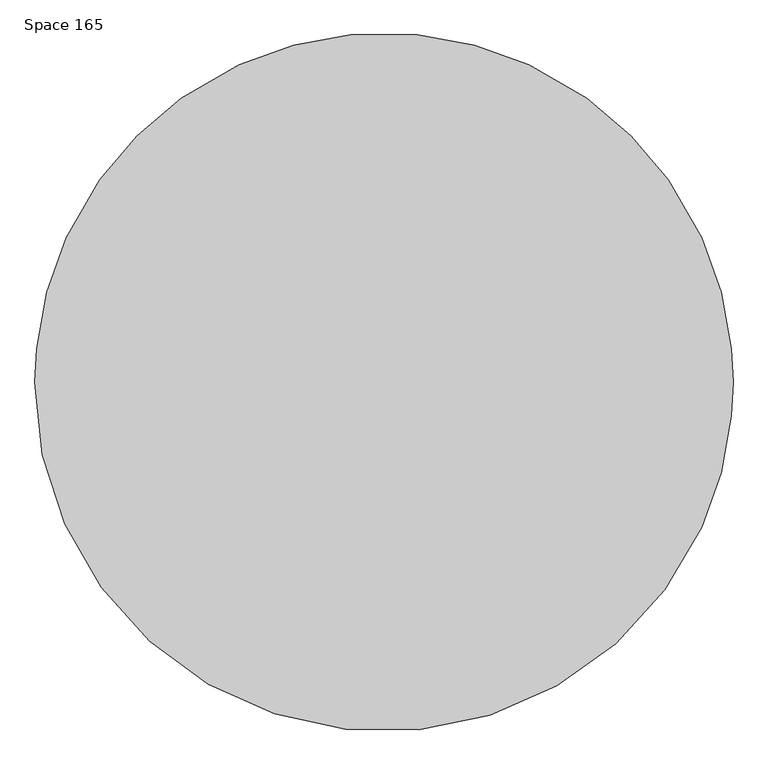
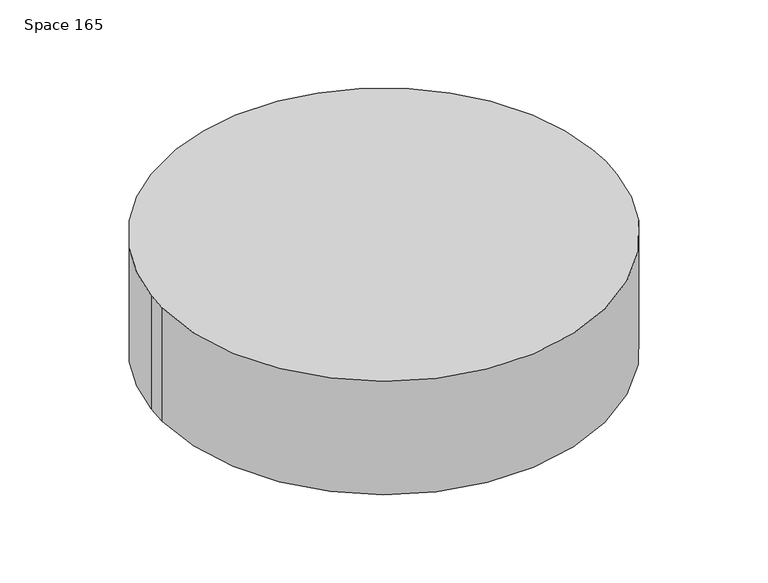
"""IFC4 building model written with IfcOpenShell, lengths in millimetres: proxy geometry, Space 165."""

from ifc_helpers import new_model, si_unit, point, frame_2d, origin, origin_with_axes, place, context, project, spatial, circle_curve, trimmed, segment, composite_curve, outline, extrude, source, transform, mapped, element, save


def space_165_78a0171c(model_context):
    return source(origin(), model_context, "Body", "SweptSolid", [
        extrude(outline(composite_curve([segment(trimmed(circle_curve(frame_2d((-24639.5440345, -26167.559635)), 5638.8), [point((-30278.3440345, -26167.559635))], [point((-30252.3841179, -25627.1046057))], False, "CARTESIAN"), True, "CONTINUOUS"), segment(trimmed(circle_curve(frame_2d((-24639.5440345, -26167.559635)), 5638.8), [point((-30252.3841179, -25627.1046057))], [point((-29770.6336487, -23829.1873783))], False, "CARTESIAN"), True, "CONTINUOUS"), segment(trimmed(circle_curve(frame_2d((-24639.5440345, -26167.559635)), 5638.8), [point((-29770.6336487, -23829.1873783))], [point((-29230.1786194, -22893.0918084))], False, "CARTESIAN"), True, "CONTINUOUS"), segment(trimmed(circle_curve(frame_2d((-24639.5440345, -26167.559635)), 5638.8), [point((-29230.1786194, -22893.0918084))], [point((-27914.0118612, -21576.9250501))], False, "CARTESIAN"), True, "CONTINUOUS"), segment(trimmed(circle_curve(frame_2d((-24639.5440345, -26167.559635)), 5638.8), [point((-27914.0118612, -21576.9250501))], [point((-26977.9162912, -21036.4700208))], False, "CARTESIAN"), True, "CONTINUOUS"), segment(trimmed(circle_curve(frame_2d((-24639.5440345, -26167.559635)), 5638.8), [point((-26977.9162912, -21036.4700208))], [point((-25179.9990638, -20554.7195517))], False, "CARTESIAN"), True, "CONTINUOUS"), segment(trimmed(circle_curve(frame_2d((-24639.5440345, -26167.559635)), 5638.8), [point((-25179.9990638, -20554.7195517))], [point((-24099.0890052, -20554.7195517))], False, "CARTESIAN"), True, "CONTINUOUS"), segment(trimmed(circle_curve(frame_2d((-24639.5440345, -26167.559635)), 5638.8), [point((-24099.0890052, -20554.7195517))], [point((-22301.1717778, -21036.4700208))], False, "CARTESIAN"), True, "CONTINUOUS"), segment(trimmed(circle_curve(frame_2d((-24639.5440345, -26167.559635)), 5638.8), [point((-22301.1717778, -21036.4700208))], [point((-21365.0762078, -21576.9250501))], False, "CARTESIAN"), True, "CONTINUOUS"), segment(trimmed(circle_curve(frame_2d((-24639.5440345, -26167.559635)), 5638.8), [point((-21365.0762078, -21576.9250501))], [point((-20048.9094496, -22893.0918084))], False, "CARTESIAN"), True, "CONTINUOUS"), segment(trimmed(circle_curve(frame_2d((-24639.5440345, -26167.559635)), 5638.8), [point((-20048.9094496, -22893.0918084))], [point((-19508.4544203, -23829.1873783))], False, "CARTESIAN"), True, "CONTINUOUS"), segment(trimmed(circle_curve(frame_2d((-24639.5440345, -26167.559635)), 5638.8), [point((-19508.4544203, -23829.1873783))], [point((-19026.7039512, -25627.1046057))], False, "CARTESIAN"), True, "CONTINUOUS"), segment(trimmed(circle_curve(frame_2d((-24639.5440345, -26167.559635)), 5638.8), [point((-19026.7039512, -25627.1046057))], [point((-19000.7440345, -26167.559635))], False, "CARTESIAN"), True, "CONTINUOUS"), segment(trimmed(circle_curve(frame_2d((-24639.5440345, -26167.559635)), 5638.8), [point((-19000.7440345, -26167.559635))], [point((-19026.7039512, -26708.0146643))], False, "CARTESIAN"), True, "CONTINUOUS"), segment(trimmed(circle_curve(frame_2d((-24639.5440345, -26167.559635)), 5638.8), [point((-19026.7039512, -26708.0146643))], [point((-19508.4544203, -28505.9318917))], False, "CARTESIAN"), True, "CONTINUOUS"), segment(trimmed(circle_curve(frame_2d((-24639.5440345, -26167.559635)), 5638.8), [point((-19508.4544203, -28505.9318917))], [point((-30278.3440345, -26167.559635))], False, "CARTESIAN"), True, "CONTINUOUS")], self_intersect=False)), origin_with_axes(), (0.0, 0.0, 1.0), 3048.0),
    ])


if __name__ == "__main__":
    model = new_model("IFC4")
    model_context = context("Model", 3, world=origin())
    ifc_project = project(units=[si_unit("LENGTHUNIT", "METRE", prefix="MILLI")], contexts=[model_context])
    site = spatial("IfcSite", under=ifc_project)
    building = spatial("IfcBuilding", under=site)
    placement = place(None, origin())
    space_165_shape = space_165_78a0171c(model_context)
    element("IfcBuildingElementProxy", 1, Name="Space 165", ObjectType="Space 165", at=placement, inside=building, context=model_context, shape_type="MappedRepresentation", body=[
        mapped(space_165_shape, transform((0.0, 0.0, 0.0), x_axis=(1.0, 0.0, 0.0), y_axis=(0.0, 1.0, 0.0), z_axis=(0.0, 0.0, 1.0))),
    ])
    save(model, "model.ifc")

# Revit data of these elements
# Element 1 (IfcBuildingElementProxy, "Space 165")
#   Materials on its faces: "Render Material 255-255-255"
# Materials
#   "Render Material 255-255-255": class "Unassigned", colour RGB 255 255 255, transparency 0
